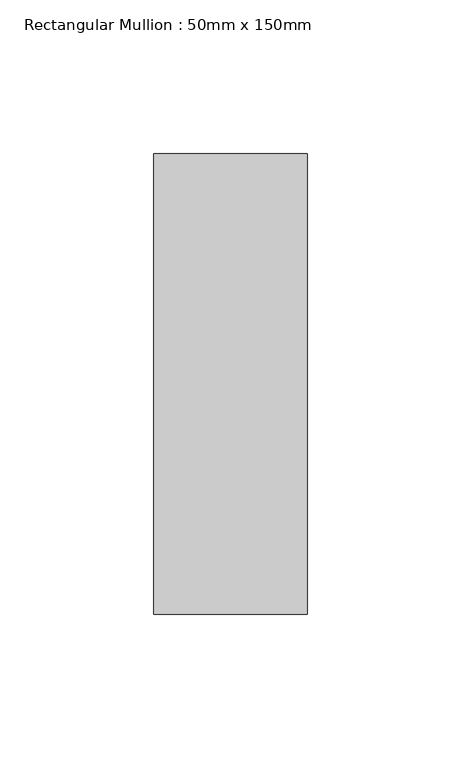
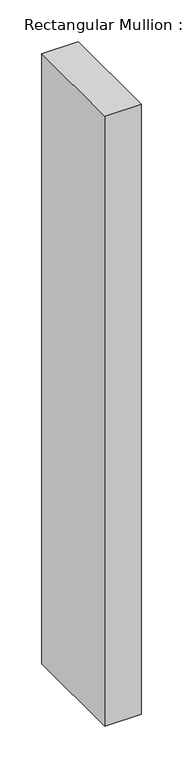
"""IFC4 building model written with IfcOpenShell, lengths in millimetres: member geometry, Rectangular Mullion : 50mm x 150mm."""

from ifc_helpers import new_model, si_unit, frame, origin, place, context, project, spatial, polyline, outline, extrude, source, transform, mapped, element, save


def rectangular_mullion_50mm_x_150mm_76640734(model_context):
    return source(origin(), model_context, "Body", "SweptSolid", [
        extrude(outline(polyline([(0.0, 75.0), (0.0, -75.0), (-50.0, -75.0), (-50.0, 75.0), (0.0, 75.0)])), frame((0.0, 0.0, -887.8787879), z_axis=(0.0, 0.0, 1.0), x_axis=(1.0, 0.0, 0.0)), (0.0, 0.0, 1.0), 887.8787879),
    ])


if __name__ == "__main__":
    model = new_model("IFC4")
    model_context = context("Model", 3, world=origin())
    ifc_project = project(units=[si_unit("LENGTHUNIT", "METRE", prefix="MILLI")], contexts=[model_context])
    site = spatial("IfcSite", under=ifc_project)
    building = spatial("IfcBuilding", under=site)
    placement = place(None, origin())
    rectangular_mullion_50mm_x_150mm_shape = rectangular_mullion_50mm_x_150mm_76640734(model_context)
    element("IfcMember", 1, ObjectType="Rectangular Mullion : 50mm x 150mm", at=placement, inside=building, context=model_context, shape_type="MappedRepresentation", body=[
        mapped(rectangular_mullion_50mm_x_150mm_shape, transform((0.0, 0.0, 0.0), x_axis=(1.0, 0.0, 0.0), y_axis=(0.0, 1.0, 0.0), z_axis=(0.0, 0.0, 1.0))),
    ])
    save(model, "model.ifc")

# Revit data of these elements
# Type "Rectangular Mullion : 50mm x 150mm"
#   built-in parameter 1007304 = 0.492126 (stored number, unit not read)
#   built-in parameter 1007301 = 0.082021 (stored number, unit not read)
#   built-in parameter 1007300 = 0.082021 (stored number, unit not read)
# Element 1 (IfcMember, "Rectangular Mullion : 50mm x 150mm")
#   Materials on its faces: "Aluminum"
# Materials
#   "Aluminum": class "Metal", colour RGB 244 244 244, transparency 0, Description = "Aluminum 6061", Cost = 0
